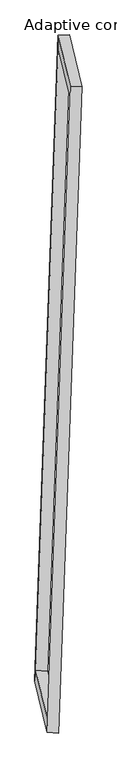
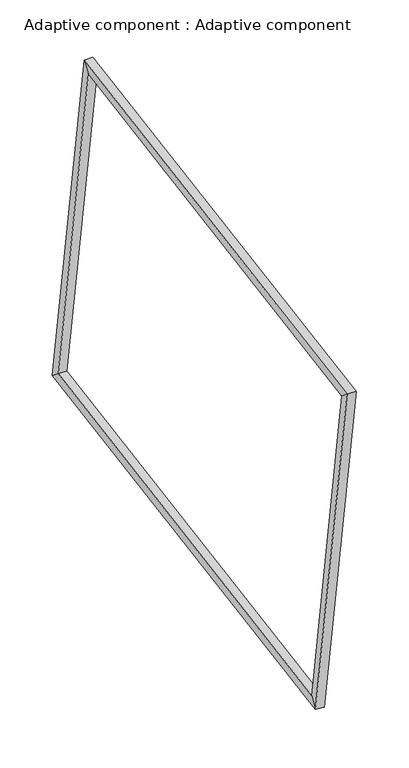
"""IFC4 building model written with IfcOpenShell, lengths in millimetres: proxy geometry, Adaptive component : Adaptive component."""

from ifc_helpers import new_model, si_unit, origin, place, context, project, spatial, faceted_brep, source, transform, mapped, element, save


def adaptive_component_adaptive_component_5d1273cf(model_context):
    return source(origin(), model_context, "Body", "Brep", [
        faceted_brep([(77.477628, 1239.6435582, 2855.5297072), (142.5064345, 1239.268994, 2855.7784581), (73.3494746, 1527.7234886, 225.3605113), (8.4244872, 1527.6650217, 229.0605727), (75.4351557, 1182.1105929, 2783.8928566), (9.7767625, 1455.9725243, 286.5445645), (140.4639622, 1181.7360287, 2784.1416076), (74.7017498, 1456.0309912, 282.8445031), (-56.9546292, -2081.9688231, -167.0564189), (-121.7370992, -2078.0792662, -162.9271599), (-115.7246994, -2020.6767075, -91.4089842), (-50.9422294, -2024.5662644, -95.5382432), (12.2023308, -2370.4233177, 2463.3615279), (-52.6839584, -2366.1007298, 2463.5419746), (-50.0663062, -2294.538639, 2405.9393079), (14.819983, -2298.8612269, 2405.7588612)], [[[0, 1, 2, 3]], [[4, 0, 3, 5]], [[6, 4, 5, 7]], [[1, 6, 7, 2]], [[3, 2, 8, 9]], [[5, 3, 9, 10]], [[7, 5, 10, 11]], [[2, 7, 11, 8]], [[9, 8, 12, 13]], [[10, 9, 13, 14]], [[11, 10, 14, 15]], [[8, 11, 15, 12]], [[13, 12, 1, 0]], [[14, 13, 0, 4]], [[15, 14, 4, 6]], [[12, 15, 6, 1]]]),
    ])


if __name__ == "__main__":
    model = new_model("IFC4")
    model_context = context("Model", 3, world=origin())
    ifc_project = project(units=[si_unit("LENGTHUNIT", "METRE", prefix="MILLI")], contexts=[model_context])
    site = spatial("IfcSite", under=ifc_project)
    building = spatial("IfcBuilding", under=site)
    placement = place(None, origin())
    adaptive_component_adaptive_component_shape = adaptive_component_adaptive_component_5d1273cf(model_context)
    element("IfcBuildingElementProxy", 1, Name="Adaptive component : Adaptive component", ObjectType="Adaptive component : Adaptive component", at=placement, inside=building, context=model_context, shape_type="MappedRepresentation", body=[
        mapped(adaptive_component_adaptive_component_shape, transform((0.0, 0.0, 0.0), x_axis=(1.0, 0.0, 0.0), y_axis=(0.0, 1.0, 0.0), z_axis=(0.0, 0.0, 1.0))),
    ])
    save(model, "model.ifc")

# Revit data of these elements
# Type "Adaptive component : Adaptive component"
#   r [instance default] = 2063.125 mm
#   2r [instance default] = 4126.251 mm
#   Number [instance default] = 5
#   Default Elevation = 0
# Element 1 (IfcBuildingElementProxy, "Adaptive component : Adaptive component")
#   r = 2154.597 mm
#   2r = 4309.194 mm
#   Number = 8
